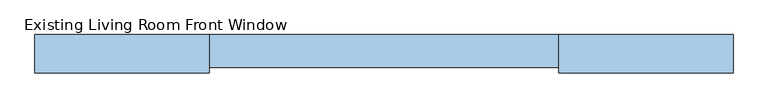
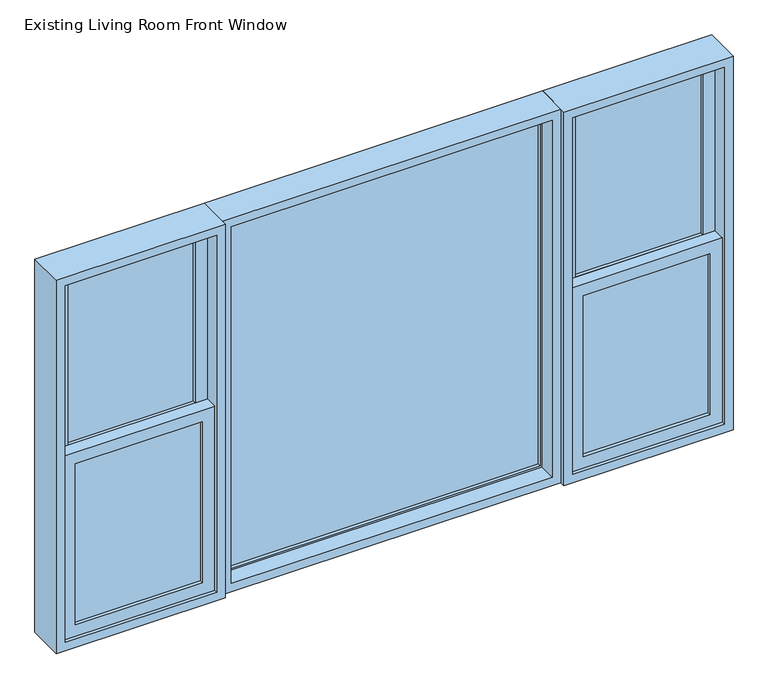
"""IFC4 building model written with IfcOpenShell, lengths in millimetres: window geometry, Existing Living Room Front Window."""

from ifc_helpers import new_model, si_unit, frame, origin, place, context, project, spatial, polyline, outline, extrude, faceted_brep, source, transform, mapped, element, save


def existing_living_room_front_window_f9ce2922(model_context):
    return source(origin(), model_context, "Body", "SolidModel", [
        extrude(outline(polyline([(-1143.0, 106.3625), (-685.8, 106.3625), (-685.8, 100.0125), (-1143.0, 100.0125), (-1143.0, 106.3625)])), frame((0.0, 0.0, 990.6), z_axis=(0.0, 0.0, 1.0), x_axis=(1.0, 0.0, 0.0)), (0.0, 0.0, 1.0), 612.775),
        extrude(outline(polyline([(-685.8, 93.6625), (-685.8, 87.3125), (-1143.0, 87.3125), (-1143.0, 93.6625), (-685.8, 93.6625)])), frame((0.0, 0.0, 990.6), z_axis=(0.0, 0.0, 1.0), x_axis=(1.0, 0.0, 0.0)), (0.0, 0.0, 1.0), 612.775),
        extrude(outline(polyline([(-1143.0, 150.8125), (-685.8, 150.8125), (-685.8, 144.4625), (-1143.0, 144.4625), (-1143.0, 150.8125)])), frame((0.0, 0.0, 1647.825), z_axis=(0.0, 0.0, 1.0), x_axis=(1.0, 0.0, 0.0)), (0.0, 0.0, 1.0), 612.775),
        extrude(outline(polyline([(-685.8, 138.1125), (-685.8, 131.7625), (-1143.0, 131.7625), (-1143.0, 138.1125), (-685.8, 138.1125)])), frame((0.0, 0.0, 1647.825), z_axis=(0.0, 0.0, 1.0), x_axis=(1.0, 0.0, 0.0)), (0.0, 0.0, 1.0), 612.775),
        extrude(outline(polyline([(1647.825, -641.35), (1647.825, -1187.45), (946.15, -1187.45), (946.15, -641.35), (1647.825, -641.35)]), holes=[polyline([(1603.375, -1143.0), (1603.375, -685.8), (990.6, -685.8), (990.6, -1143.0), (1603.375, -1143.0)])]), frame((0.0, 74.6125, 0.0), z_axis=(0.0, 1.0, 0.0), x_axis=(0.0, 0.0, 1.0)), (0.0, 0.0, 1.0), 44.45),
        extrude(outline(polyline([(2305.05, -641.35), (2305.05, -1187.45), (1603.375, -1187.45), (1603.375, -641.35), (2305.05, -641.35)]), holes=[polyline([(2260.6, -1143.0), (2260.6, -685.8), (1647.825, -685.8), (1647.825, -1143.0), (2260.6, -1143.0)])]), frame((0.0, 119.0625, 0.0), z_axis=(0.0, 1.0, 0.0), x_axis=(0.0, 0.0, 1.0)), (0.0, 0.0, 1.0), 44.45),
        extrude(outline(polyline([(2336.8, -609.6), (2336.8, -1219.2), (914.4, -1219.2), (914.4, -609.6), (2336.8, -609.6)]), holes=[polyline([(2305.05, -1187.45), (2305.05, -641.35), (946.15, -641.35), (946.15, -1187.45), (2305.05, -1187.45)])]), frame((0.0, 61.9125, 0.0), z_axis=(0.0, 1.0, 0.0), x_axis=(0.0, 0.0, 1.0)), (0.0, 0.0, 1.0), 133.35),
        extrude(outline(polyline([(685.8, 106.3625), (1143.0, 106.3625), (1143.0, 100.0125), (685.8, 100.0125), (685.8, 106.3625)])), frame((0.0, 0.0, 990.6), z_axis=(0.0, 0.0, 1.0), x_axis=(1.0, 0.0, 0.0)), (0.0, 0.0, 1.0), 612.775),
        extrude(outline(polyline([(1143.0, 93.6625), (1143.0, 87.3125), (685.8, 87.3125), (685.8, 93.6625), (1143.0, 93.6625)])), frame((0.0, 0.0, 990.6), z_axis=(0.0, 0.0, 1.0), x_axis=(1.0, 0.0, 0.0)), (0.0, 0.0, 1.0), 612.775),
        extrude(outline(polyline([(685.8, 150.8125), (1143.0, 150.8125), (1143.0, 144.4625), (685.8, 144.4625), (685.8, 150.8125)])), frame((0.0, 0.0, 1647.825), z_axis=(0.0, 0.0, 1.0), x_axis=(1.0, 0.0, 0.0)), (0.0, 0.0, 1.0), 612.775),
        extrude(outline(polyline([(1143.0, 138.1125), (1143.0, 131.7625), (685.8, 131.7625), (685.8, 138.1125), (1143.0, 138.1125)])), frame((0.0, 0.0, 1647.825), z_axis=(0.0, 0.0, 1.0), x_axis=(1.0, 0.0, 0.0)), (0.0, 0.0, 1.0), 612.775),
        extrude(outline(polyline([(1647.825, 1187.45), (1647.825, 641.35), (946.15, 641.35), (946.15, 1187.45), (1647.825, 1187.45)]), holes=[polyline([(1603.375, 685.8), (1603.375, 1143.0), (990.6, 1143.0), (990.6, 685.8), (1603.375, 685.8)])]), frame((0.0, 74.6125, 0.0), z_axis=(0.0, 1.0, 0.0), x_axis=(0.0, 0.0, 1.0)), (0.0, 0.0, 1.0), 44.45),
        extrude(outline(polyline([(2305.05, 1187.45), (2305.05, 641.35), (1603.375, 641.35), (1603.375, 1187.45), (2305.05, 1187.45)]), holes=[polyline([(2260.6, 685.8), (2260.6, 1143.0), (1647.825, 1143.0), (1647.825, 685.8), (2260.6, 685.8)])]), frame((0.0, 119.0625, 0.0), z_axis=(0.0, 1.0, 0.0), x_axis=(0.0, 0.0, 1.0)), (0.0, 0.0, 1.0), 44.45),
        extrude(outline(polyline([(2336.8, 1219.2), (2336.8, 609.6), (914.4, 609.6), (914.4, 1219.2), (2336.8, 1219.2)]), holes=[polyline([(2305.05, 641.35), (2305.05, 1187.45), (946.15, 1187.45), (946.15, 641.35), (2305.05, 641.35)])]), frame((0.0, 61.9125, 0.0), z_axis=(0.0, 1.0, 0.0), x_axis=(0.0, 0.0, 1.0)), (0.0, 0.0, 1.0), 133.35),
        extrude(outline(polyline([(-571.5, 176.2125), (571.5, 176.2125), (571.5, 169.8625), (-571.5, 169.8625), (-571.5, 176.2125)])), frame((0.0, 0.0, 952.5), z_axis=(0.0, 0.0, 1.0), x_axis=(1.0, 0.0, 0.0)), (0.0, 0.0, 1.0), 1346.2),
        extrude(outline(polyline([(571.5, 157.1625), (-571.5, 157.1625), (-571.5, 163.5125), (571.5, 163.5125), (571.5, 157.1625)])), frame((0.0, 0.0, 952.5), z_axis=(0.0, 0.0, 1.0), x_axis=(1.0, 0.0, 0.0)), (0.0, 0.0, 1.0), 1346.2),
        extrude(outline(polyline([(927.1, -596.9), (927.1, 596.9), (2324.1, 596.9), (2324.1, -596.9), (927.1, -596.9)]), holes=[polyline([(952.5, 571.5), (952.5, -571.5), (2298.7, -571.5), (2298.7, 571.5), (952.5, 571.5)])]), frame((0.0, 144.4625, 0.0), z_axis=(0.0, 1.0, 0.0), x_axis=(0.0, 0.0, 1.0)), (0.0, 0.0, 1.0), 44.45),
        faceted_brep([(-609.6, 80.9625, 2336.8), (609.6, 80.9625, 2336.8), (609.6, 195.2625, 2336.8), (-609.6, 195.2625, 2336.8), (609.6, 80.9625, 914.4), (609.6, 195.2625, 914.4), (-609.6, 80.9625, 914.4), (-609.6, 195.2625, 914.4), (-577.85, 80.9625, 2305.05), (577.85, 80.9625, 2305.05), (577.85, 80.9625, 946.15), (-577.85, 80.9625, 946.15), (596.9, 195.2625, 2324.1), (-596.9, 195.2625, 2324.1), (-596.9, 195.2625, 927.1), (596.9, 195.2625, 927.1), (-577.85, 144.4625, 2305.05), (577.85, 144.4625, 2305.05), (596.9, 144.4625, 2324.1), (-596.9, 144.4625, 2324.1), (577.85, 144.4625, 946.15), (596.9, 144.4625, 927.1), (-577.85, 144.4625, 946.15), (-596.9, 144.4625, 927.1)], [[[0, 1, 2, 3]], [[1, 4, 5, 2]], [[4, 6, 7, 5]], [[1, 0, 6, 4], [8, 9, 10, 11]], [[6, 0, 3, 7]], [[3, 2, 5, 7], [12, 13, 14, 15]], [[16, 17, 9, 8]], [[13, 12, 18, 19]], [[17, 20, 10, 9]], [[12, 15, 21, 18]], [[20, 22, 11, 10]], [[15, 14, 23, 21]], [[22, 16, 8, 11]], [[19, 18, 21, 23], [17, 16, 22, 20]], [[14, 13, 19, 23]]]),
    ])


if __name__ == "__main__":
    model = new_model("IFC4")
    model_context = context("Model", 3, world=origin())
    ifc_project = project(units=[si_unit("LENGTHUNIT", "METRE", prefix="MILLI")], contexts=[model_context])
    site = spatial("IfcSite", under=ifc_project)
    building = spatial("IfcBuilding", under=site)
    placement = place(None, origin())
    existing_living_room_front_window_shape = existing_living_room_front_window_f9ce2922(model_context)
    element("IfcWindow", 1, ObjectType="Existing Living Room Front Window : (2) 2'-0\" x 4'-8\" DH + 4'-0\" x 4'-8\" FX", at=placement, inside=building, context=model_context, shape_type="MappedRepresentation", body=[
        mapped(existing_living_room_front_window_shape, transform((0.0, 0.0, 0.0), x_axis=(1.0, 0.0, 0.0), y_axis=(0.0, 1.0, 0.0), z_axis=(0.0, 0.0, 1.0))),
    ])
    save(model, "model.ifc")

# Revit data of these elements
# Type "Existing Living Room Front Window : (2) 2'-0\" x 4'-8\" DH + 4'-0\" x 4'-8\" FX"
#   Type Mark = "21"
#   Analytic Construction = "<None>"
#   Window Inset = 0' - 0 3/4"
#   Side Window Width = 2' - 0"
#   Side Window Location = 2' - 0"
#   Middle Window Width = 4' - 0"
#   Height = 4' - 8"
#   Default Sill Height = 3' - 0"
#   Width = 8' - 0"
#   Top Muntin Visibility = yes
#   Interior Trim Visibility [instance default] = yes
#   Fixed Muntin Visibility = no
#   Exterior Trim Visibility [instance default] = yes
#   Define Thermal Properties by = 1
#   Bottom Muntin Visibility = yes
#   Sash Material = Sash
#   Interior Trim = Trim-Window-Interior-Flat : Picture Frame
#   Interior Trim Material = Wood - Stained
#   Interior Frame Material = Wood - Stained
#   Glass Pane Material = Glass
#   Exterior Trim Material = Clad - White
#   Exterior Trim = Trim-Window-Exterior-Flat : with Sill
#   Exterior Frame Material = Clad - White
#   Rough Width = 0
#   Rough Height = 0
#   Wall Closure = (empty or 0)
# Element 1 (IfcWindow, "Existing Living Room Front Window : (2) 2'-0\" x 4'-8\" DH + 4'-0\" x 4'-8\" FX")
#   Materials on its faces: "Wood - Stained", "Glass", "Clad - White"
# Materials
#   "Sash": class "Wood", colour RGB 224 178 126, transparency 0, Cost = 0
#   "Wood - Stained": class "Wood", colour RGB 224 178 126, transparency 0, Cost = 0
#   "Glass": class "Glass", colour RGB 0 128 192, transparency 0.75, Description = "Soda Lime Glass", Cost = 0
#   "Clad - White": class "Wood", colour RGB 242 242 238, transparency 0, Cost = 0
